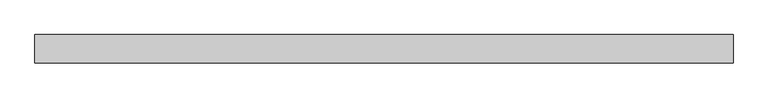
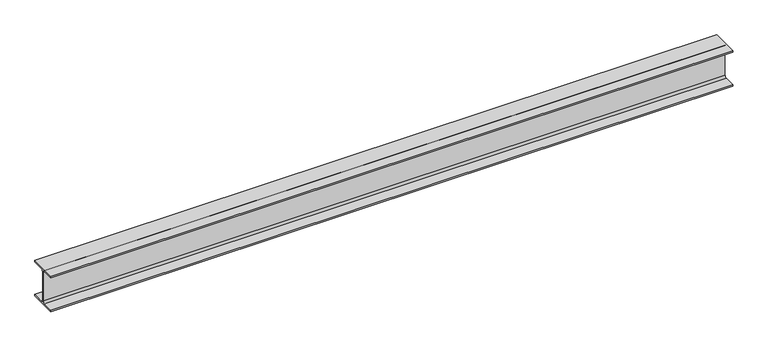
"""IFC4 building model written with IfcOpenShell, lengths in millimetres: beam geometry, 0912_Steel Framing_H-KSD3502 : H_SB_ASB_H-340x250x9x14."""

import ifcopenshell
import ifcopenshell.guid

model = None  # the IFC model being written
_history = None  # IfcOwnerHistory: only IFC2X3 demands one
_inside = {}  # id of a spatial element -> (the spatial element, [elements in it])
_under = {}  # id of a project, library or spatial element -> (it, [spatial elements below it])
_declared = {}  # id of a project -> (the project, [libraries it declares])
_typed = {}  # id of a type object -> (the type object, [elements of that type])
_made_of = {}  # id of a material, layer set ... -> (it, [elements and type objects made of it])


def new_model(schema):
    """Start an empty IFC model of exactly this schema.

    Asked for "IFC4X3", IfcOpenShell would pick the latest addendum, in which some entities
    have other attributes; the version numbers below select the first issue.
    IFC2X3 requires an IfcOwnerHistory on every rooted entity: one is made here for all.
    """
    global model, _history
    if schema == "IFC4X3":
        model = ifcopenshell.file(schema_version=(4, 3, 0, 0))
    else:
        model = ifcopenshell.file(schema=schema)
    _inside.clear()
    _under.clear()
    _declared.clear()
    _typed.clear()
    _made_of.clear()
    _history = None
    if model.schema == "IFC2X3":
        org = make("IfcOrganization", Name="unknown")
        user = make(
            "IfcPersonAndOrganization",
            ThePerson=make("IfcPerson", FamilyName="unknown"),
            TheOrganization=org,
        )
        app = make(
            "IfcApplication",
            ApplicationDeveloper=org,
            Version="unknown",
            ApplicationFullName="unknown",
            ApplicationIdentifier="unknown",
        )
        _history = make(
            "IfcOwnerHistory",
            OwningUser=user,
            OwningApplication=app,
            ChangeAction="ADDED",
            CreationDate=0,
        )
    return model


def make(cls, **values):
    """One entity of the class cls with the attributes given. An attribute that is None is left unset."""
    return model.create_entity(
        cls, **{name: value for name, value in values.items() if value is not None}
    )


def rooted(cls, **values):
    """An entity with a GlobalId (a new one), such as an element, a storey or a relation."""
    return make(cls, GlobalId=ifcopenshell.guid.new(), OwnerHistory=_history, **values)


def si_unit(unit_type, name, prefix=None):
    """IfcSIUnit, for example si_unit("LENGTHUNIT", "METRE", prefix="MILLI")."""
    return make("IfcSIUnit", UnitType=unit_type, Prefix=prefix, Name=name)


def assignment(units):
    """IfcUnitAssignment: the units of a project."""
    return None if units is None else make("IfcUnitAssignment", Units=units)


def point(xyz):
    """IfcCartesianPoint."""
    return None if xyz is None else make("IfcCartesianPoint", Coordinates=xyz)


def direction(xyz):
    """IfcDirection."""
    return None if xyz is None else make("IfcDirection", DirectionRatios=xyz)


def frame(location, z_axis=None, x_axis=None):
    """IfcAxis2Placement3D, a coordinate frame: its origin and axes. An axis left out is left unset."""
    return make(
        "IfcAxis2Placement3D",
        Location=point(location),
        Axis=direction(z_axis),
        RefDirection=direction(x_axis),
    )


def frame_2d(location, x_axis=None):
    """IfcAxis2Placement2D, a coordinate frame in the plane: its origin and x axis."""
    return make(
        "IfcAxis2Placement2D", Location=point(location), RefDirection=direction(x_axis)
    )


def origin():
    """The frame at (0, 0, 0) with its axes left unset."""
    return frame((0.0, 0.0, 0.0))


def place(relative_to, where):
    """IfcLocalPlacement: puts the frame where relative to a parent placement (None: the world)."""
    return make(
        "IfcLocalPlacement", PlacementRelTo=relative_to, RelativePlacement=where
    )


def context(
    kind, dimensions, precision=None, world=None, true_north=None, identifier=None
):
    """IfcGeometricRepresentationContext, for example the 3D "Model" context."""
    return make(
        "IfcGeometricRepresentationContext",
        ContextIdentifier=identifier,
        ContextType=kind,
        CoordinateSpaceDimension=dimensions,
        Precision=precision,
        WorldCoordinateSystem=world,
        TrueNorth=true_north,
    )


def project(units=None, contexts=None):
    """IfcProject with its units and contexts."""
    return rooted(
        "IfcProject",
        Name="project",
        RepresentationContexts=contexts,
        UnitsInContext=assignment(units),
    )


def spatial(cls, under=None, at=None, **own):
    """A site, building, storey or space (cls), placed at a placement, below another one or the project."""
    s = rooted(cls, ObjectPlacement=at, **own)
    if under is not None:
        _under.setdefault(under.id(), (under, []))[1].append(s)
    return s


def polyline(points):
    """IfcPolyline through the points."""
    return make("IfcPolyline", Points=[point(p) for p in points])


def circle_curve(where, radius):
    """IfcCircle in the frame where."""
    return make("IfcCircle", Position=where, Radius=radius)


def trimmed(basis, trim1, trim2, sense, master):
    """IfcTrimmedCurve: the piece of a basis curve between two trims."""
    return make(
        "IfcTrimmedCurve",
        BasisCurve=basis,
        Trim1=trim1,
        Trim2=trim2,
        SenseAgreement=sense,
        MasterRepresentation=master,
    )


def segment(curve, same_sense, transition):
    """IfcCompositeCurveSegment."""
    return make(
        "IfcCompositeCurveSegment",
        Transition=transition,
        SameSense=same_sense,
        ParentCurve=curve,
    )


def composite_curve(segments, self_intersect=None):
    """IfcCompositeCurve: segments joined end to end."""
    return make("IfcCompositeCurve", Segments=segments, SelfIntersect=self_intersect)


def outline(outer, holes=None, kind="AREA"):
    """IfcArbitraryClosedProfileDef: a profile drawn as a closed curve; with holes, ...WithVoids."""
    if holes is None:
        return make("IfcArbitraryClosedProfileDef", ProfileType=kind, OuterCurve=outer)
    return make(
        "IfcArbitraryProfileDefWithVoids",
        ProfileType=kind,
        OuterCurve=outer,
        InnerCurves=holes,
    )


def extrude(swept, where, along, depth):
    """IfcExtrudedAreaSolid: the profile swept, set in the frame where, extruded along a direction by depth."""
    return make(
        "IfcExtrudedAreaSolid",
        SweptArea=swept,
        Position=where,
        ExtrudedDirection=direction(along),
        Depth=depth,
    )


def shape(context_of_items, identifier, shape_type, items):
    """IfcShapeRepresentation: the items that make up one representation, for example the "Body"."""
    return make(
        "IfcShapeRepresentation",
        ContextOfItems=context_of_items,
        RepresentationIdentifier=identifier,
        RepresentationType=shape_type,
        Items=items,
    )


def source(mapping_origin, context_of_items, identifier, shape_type, items):
    """IfcRepresentationMap: a shape defined once, which mapped items show again and again."""
    return make(
        "IfcRepresentationMap",
        MappingOrigin=mapping_origin,
        MappedRepresentation=shape(context_of_items, identifier, shape_type, items),
    )


def transform(
    local_origin,
    x_axis=None,
    y_axis=None,
    z_axis=None,
    scale=None,
    scale2=None,
    scale3=None,
    uniform=True,
):
    """IfcCartesianTransformationOperator3D, or its non-uniform kind. x_axis, y_axis, z_axis: its Axis1, 2, 3."""
    if uniform:
        return make(
            "IfcCartesianTransformationOperator3D",
            Axis1=direction(x_axis),
            Axis2=direction(y_axis),
            LocalOrigin=point(local_origin),
            Scale=scale,
            Axis3=direction(z_axis),
        )
    return make(
        "IfcCartesianTransformationOperator3DnonUniform",
        Axis1=direction(x_axis),
        Axis2=direction(y_axis),
        LocalOrigin=point(local_origin),
        Scale=scale,
        Axis3=direction(z_axis),
        Scale2=scale2,
        Scale3=scale3,
    )


def mapped(mapping_source, mapping_target):
    """IfcMappedItem: shows the shape of a source again, moved by a transform."""
    return make(
        "IfcMappedItem", MappingSource=mapping_source, MappingTarget=mapping_target
    )


def made_of(thing, what):
    """Note that an element or type object is made of a material, layer set ...; save() writes the relation."""
    if what is not None:
        _made_of.setdefault(what.id(), (what, []))[1].append(thing)
    return thing


def element(
    cls,
    number,
    at=None,
    inside=None,
    cuts=None,
    type_object=None,
    material=None,
    context=None,
    identifier="Body",
    shape_type=None,
    held_by="IfcProductDefinitionShape",
    body=None,
    shapes=None,
    **own,
):
    """One element of the class cls, such as IfcWall. Its Tag is "e" and its number.

    at: its placement. inside: the storey or other place that contains it. cuts: it is an
    opening in that element (IfcRelVoidsElement). A single representation is given by context,
    identifier, shape_type and body (its items); several are given by shapes. held_by: the class
    of the entity that holds the representations. save() writes the other relations.
    """
    e = rooted(cls, Tag="e%d" % number, ObjectPlacement=at, **own)
    if body is not None:
        shapes = [shape(context, identifier, shape_type, body)]
    if shapes is not None:
        e.Representation = make(held_by, Representations=shapes)
    if inside is not None:
        _inside.setdefault(inside.id(), (inside, []))[1].append(e)
    if cuts is not None:
        rooted(
            "IfcRelVoidsElement", RelatingBuildingElement=cuts, RelatedOpeningElement=e
        )
    if type_object is not None:
        _typed.setdefault(type_object.id(), (type_object, []))[1].append(e)
    return made_of(e, material)


def aggregate(whole, parts):
    """IfcRelAggregates: a whole, such as a stair, and the parts it consists of."""
    return rooted("IfcRelAggregates", RelatingObject=whole, RelatedObjects=parts)


def save(model, path):
    """Write the relations noted so far, then the file.

    IfcRelAggregates (storeys below a building ...), IfcRelContainedInSpatialStructure (elements
    in a storey), IfcRelDefinesByType, IfcRelAssociatesMaterial and IfcRelDeclares: one each for
    every whole, place, type object, material and project.
    """
    for whole, parts in _under.values():
        aggregate(whole, parts)
    for where, things in _inside.values():
        rooted(
            "IfcRelContainedInSpatialStructure",
            RelatedElements=things,
            RelatingStructure=where,
        )
    for kind, things in _typed.values():
        rooted("IfcRelDefinesByType", RelatedObjects=things, RelatingType=kind)
    for what, things in _made_of.values():
        rooted("IfcRelAssociatesMaterial", RelatedObjects=things, RelatingMaterial=what)
    for by, libraries in _declared.values():
        rooted("IfcRelDeclares", RelatingContext=by, RelatedDefinitions=libraries)
    model.write(path)


def beam_8c186262(model_context):
    return source(origin(), model_context, "Body", "SweptSolid", [
        extrude(outline(composite_curve([segment(polyline([(125.0, -156.0), (125.0, -170.0), (-125.0, -170.0), (-125.0, -156.0), (-24.5, -156.0)]), True, "CONTINUOUS"), segment(trimmed(circle_curve(frame_2d((-24.5, -136.0)), 20.0), [point((-24.5, -156.0))], [point((-4.5, -136.0))], True, "CARTESIAN"), True, "CONTINUOUS"), segment(polyline([(-4.5, -136.0), (-4.5, 136.0)]), True, "CONTINUOUS"), segment(trimmed(circle_curve(frame_2d((-24.5, 136.0)), 20.0), [point((-4.5, 136.0))], [point((-24.5, 156.0))], True, "CARTESIAN"), True, "CONTINUOUS"), segment(polyline([(-24.5, 156.0), (-125.0, 156.0), (-125.0, 170.0), (125.0, 170.0), (125.0, 156.0), (24.5, 156.0)]), True, "CONTINUOUS"), segment(trimmed(circle_curve(frame_2d((24.5, 136.0)), 20.0), [point((24.5, 156.0))], [point((4.5, 136.0))], True, "CARTESIAN"), True, "CONTINUOUS"), segment(polyline([(4.5, 136.0), (4.5, -136.0)]), True, "CONTINUOUS"), segment(trimmed(circle_curve(frame_2d((24.5, -136.0)), 20.0), [point((4.5, -136.0))], [point((24.5, -156.0))], True, "CARTESIAN"), True, "CONTINUOUS"), segment(polyline([(24.5, -156.0), (125.0, -156.0)]), True, "CONTINUOUS")], self_intersect=False)), frame((-3087.3, 0.0, 0.0), z_axis=(1.0, 0.0, 0.0), x_axis=(0.0, 1.0, 0.0)), (0.0, 0.0, 1.0), 6174.6),
    ])


if __name__ == "__main__":
    model = new_model("IFC4")
    model_context = context("Model", 3, world=origin())
    ifc_project = project(units=[si_unit("LENGTHUNIT", "METRE", prefix="MILLI")], contexts=[model_context])
    site = spatial("IfcSite", under=ifc_project)
    building = spatial("IfcBuilding", under=site)
    placement = place(None, origin())
    beam_shape = beam_8c186262(model_context)
    element("IfcBeam", 1, ObjectType="0912_Steel Framing_H-KSD3502 : H_SB_ASB_H-340x250x9x14", at=placement, inside=building, context=model_context, shape_type="MappedRepresentation", body=[
        mapped(beam_shape, transform((0.0, 0.0, 0.0), x_axis=(1.0, 0.0, 0.0), y_axis=(0.0, 1.0, 0.0), z_axis=(0.0, 0.0, 1.0))),
    ])
    save(model, "model.ifc")

# Revit data of these elements
# Type "0912_Steel Framing_H-KSD3502 : H_SB_ASB_H-340x250x9x14"
#   H_WM Code_1 = "S01AA002-00001 | Main Steel Structure Fabrication Work | Shelter/Building | Medium Steel - Standard (90KG/M>Weight≥30KG/M) | Material: (   )"
#   H_WM Code_2 = "S03AA028-00001 | Main Steel Structure Erection Work | Shelter/Building | Medium Steel (90KG/M>Weight≥30KG/M) | Material: (   )"
#   H_WM Code_3 = "S01AA010-00001 | Main Steel Structure Fabrication Work | Shelter/Building | Steel Painting/Coating | for Non-Fireproofed Steel Surface, Surface Preparation, Primer, Second & Final Coat | Material: (   )"
#   H_Q'ty Cal Type Tag = "SB-Q2"
#   Width = 25.0 cm
#   Web Thickness = 0.9 cm
#   Web Fillet = 2.0 cm
#   Warping Constant = 969000.0 cm⁶
#   W = 0
#   Torsional Moment of Inertia = 53.6551 cm⁴
#   Section Area = 101.5 cm²
#   Plastic Modulus weak axis = 447.0 cm³
#   Plastic Modulus strong axis = 1410.0 cm³
#   Perimeter = 1.63 m²/m
#   Nominal Weight = 79.70 kgf/m
#   Moment of Inertia weak axis = 3650.00 cm⁴
#   Moment of Inertia strong axis = 21700.00 cm⁴
#   Height = 34.0 cm
#   Flange Thickness = 1.4 cm
#   Elastic Modulus weak axis = 292.0 cm³
#   Elastic Modulus strong axis = 1280.0 cm³
#   Centroid Vertical = 17.0 cm
#   Centroid Horizontal = 12.5 cm
#   Ix = 217000000
#   Length [instance default] = 1.5240 m
#   Zx = 1410000
#   b = 0.2500 m
#   h = 0.3400 m
#   r = 0.0200 m
#   s = 0.0090 m
#   t = 0.0140 m
#   A = 0.01015 m²
#   Structural Material [instance default] = Steel, 45-345
#   Assembly Code = ""
# Element 1 (IfcBeam, "0912_Steel Framing_H-KSD3502 : H_SB_ASB_H-340x250x9x14")
#   Structural Material = none
# Materials
#   "Steel, 45-345": class "Metal", colour RGB 189 187 185, transparency 0, Description = "Steel 345 MPa", Cost = 0
